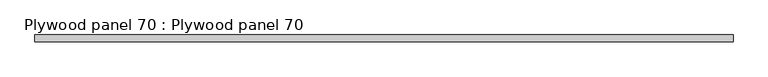
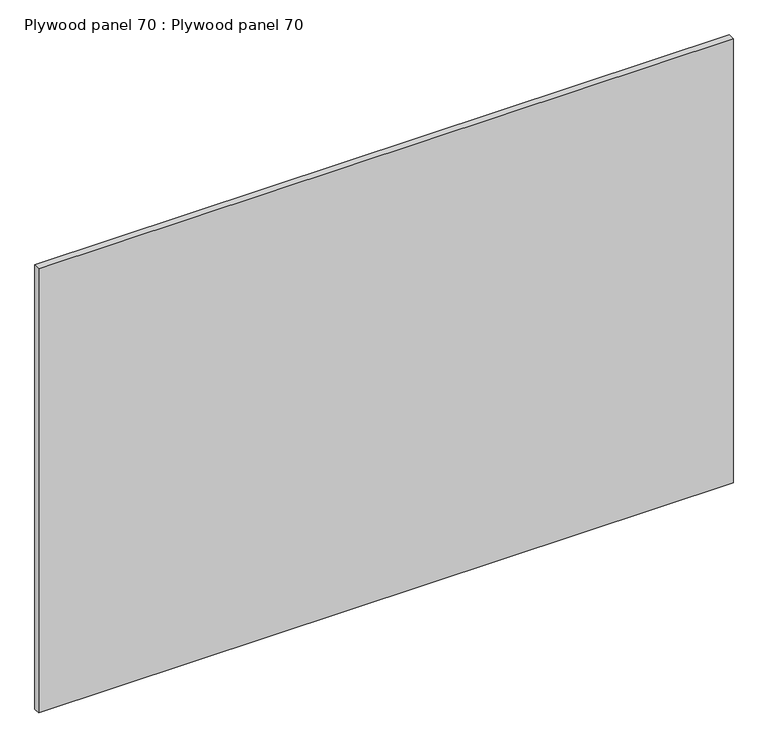
"""IFC4 building model written with IfcOpenShell, lengths in millimetres: proxy geometry, Plywood panel 70 : Plywood panel 70."""

from ifc_helpers import new_model, si_unit, frame, origin, place, context, project, spatial, polyline, outline, extrude, source, transform, mapped, element, save


def plywood_panel_70_plywood_panel_70_f1ebfc00(model_context):
    return source(origin(), model_context, "Body", "SweptSolid", [
        extrude(outline(polyline([(3694.2883192, 10417.7258229), (3694.2883192, 10436.7726979), (5694.2883192, 10436.7726979), (5694.2883192, 10417.7258229), (3694.2883192, 10417.7258229)])), frame((0.0, 0.0, 39420.546875), z_axis=(0.0, 0.0, 1.0), x_axis=(1.0, 0.0, 0.0)), (0.0, 0.0, 1.0), 1352.55),
    ])


if __name__ == "__main__":
    model = new_model("IFC4")
    model_context = context("Model", 3, world=origin())
    ifc_project = project(units=[si_unit("LENGTHUNIT", "METRE", prefix="MILLI")], contexts=[model_context])
    site = spatial("IfcSite", under=ifc_project)
    building = spatial("IfcBuilding", under=site)
    placement = place(None, origin())
    plywood_panel_70_plywood_panel_70_shape = plywood_panel_70_plywood_panel_70_f1ebfc00(model_context)
    element("IfcBuildingElementProxy", 1, Name="Plywood panel 70 : Plywood panel 70", ObjectType="Plywood panel 70 : Plywood panel 70", at=placement, inside=building, context=model_context, shape_type="MappedRepresentation", body=[
        mapped(plywood_panel_70_plywood_panel_70_shape, transform((0.0, 0.0, 0.0), x_axis=(1.0, 0.0, 0.0), y_axis=(0.0, 1.0, 0.0), z_axis=(0.0, 0.0, 1.0))),
    ])
    save(model, "model.ifc")

# Revit data of these elements
# Type "Plywood panel 70 : Plywood panel 70"
#   NameOverride = "Plywood panel"
# Element 1 (IfcBuildingElementProxy, "Plywood panel 70 : Plywood panel 70")
#   Materials on its faces: "CDX PLYWOOD - SEE STRUCTURAL DWGS"
# Materials
#   "CDX PLYWOOD - SEE STRUCTURAL DWGS": class "Unassigned", colour RGB 177 130 114, transparency 0, Cost = 0
